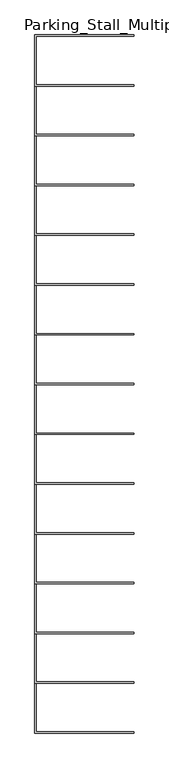
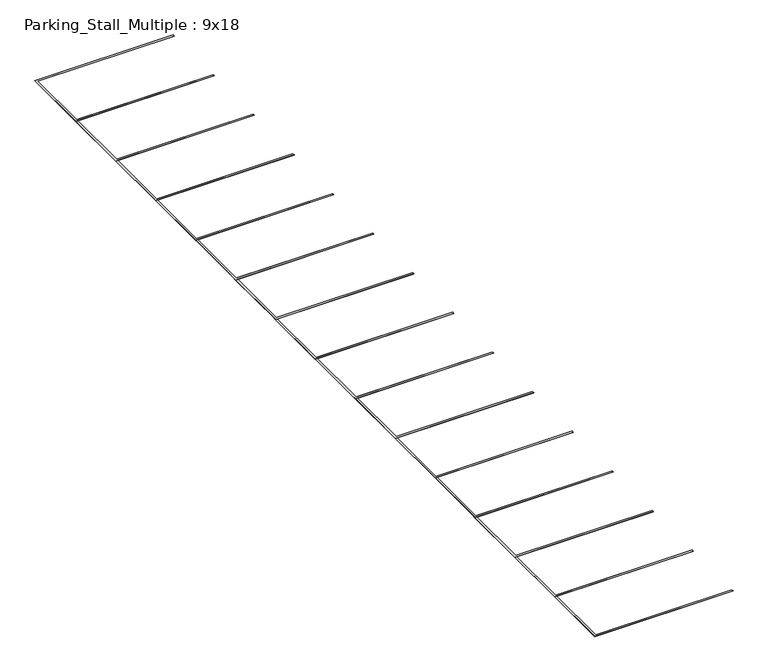
"""IFC4 building model written with IfcOpenShell, lengths in millimetres: proxy geometry, Parking_Stall_Multiple : 9x18."""

import ifcopenshell
import ifcopenshell.guid

model = None  # the IFC model being written
_history = None  # IfcOwnerHistory: only IFC2X3 demands one
_inside = {}  # id of a spatial element -> (the spatial element, [elements in it])
_under = {}  # id of a project, library or spatial element -> (it, [spatial elements below it])
_declared = {}  # id of a project -> (the project, [libraries it declares])
_typed = {}  # id of a type object -> (the type object, [elements of that type])
_made_of = {}  # id of a material, layer set ... -> (it, [elements and type objects made of it])


def new_model(schema):
    """Start an empty IFC model of exactly this schema.

    Asked for "IFC4X3", IfcOpenShell would pick the latest addendum, in which some entities
    have other attributes; the version numbers below select the first issue.
    IFC2X3 requires an IfcOwnerHistory on every rooted entity: one is made here for all.
    """
    global model, _history
    if schema == "IFC4X3":
        model = ifcopenshell.file(schema_version=(4, 3, 0, 0))
    else:
        model = ifcopenshell.file(schema=schema)
    _inside.clear()
    _under.clear()
    _declared.clear()
    _typed.clear()
    _made_of.clear()
    _history = None
    if model.schema == "IFC2X3":
        org = make("IfcOrganization", Name="unknown")
        user = make(
            "IfcPersonAndOrganization",
            ThePerson=make("IfcPerson", FamilyName="unknown"),
            TheOrganization=org,
        )
        app = make(
            "IfcApplication",
            ApplicationDeveloper=org,
            Version="unknown",
            ApplicationFullName="unknown",
            ApplicationIdentifier="unknown",
        )
        _history = make(
            "IfcOwnerHistory",
            OwningUser=user,
            OwningApplication=app,
            ChangeAction="ADDED",
            CreationDate=0,
        )
    return model


def make(cls, **values):
    """One entity of the class cls with the attributes given. An attribute that is None is left unset."""
    return model.create_entity(
        cls, **{name: value for name, value in values.items() if value is not None}
    )


def rooted(cls, **values):
    """An entity with a GlobalId (a new one), such as an element, a storey or a relation."""
    return make(cls, GlobalId=ifcopenshell.guid.new(), OwnerHistory=_history, **values)


def si_unit(unit_type, name, prefix=None):
    """IfcSIUnit, for example si_unit("LENGTHUNIT", "METRE", prefix="MILLI")."""
    return make("IfcSIUnit", UnitType=unit_type, Prefix=prefix, Name=name)


def assignment(units):
    """IfcUnitAssignment: the units of a project."""
    return None if units is None else make("IfcUnitAssignment", Units=units)


def point(xyz):
    """IfcCartesianPoint."""
    return None if xyz is None else make("IfcCartesianPoint", Coordinates=xyz)


def direction(xyz):
    """IfcDirection."""
    return None if xyz is None else make("IfcDirection", DirectionRatios=xyz)


def frame(location, z_axis=None, x_axis=None):
    """IfcAxis2Placement3D, a coordinate frame: its origin and axes. An axis left out is left unset."""
    return make(
        "IfcAxis2Placement3D",
        Location=point(location),
        Axis=direction(z_axis),
        RefDirection=direction(x_axis),
    )


def origin():
    """The frame at (0, 0, 0) with its axes left unset."""
    return frame((0.0, 0.0, 0.0))


def origin_with_axes():
    """The frame at (0, 0, 0) with the z axis (0, 0, 1) and the x axis (1, 0, 0) written out."""
    return frame((0.0, 0.0, 0.0), z_axis=(0.0, 0.0, 1.0), x_axis=(1.0, 0.0, 0.0))


def place(relative_to, where):
    """IfcLocalPlacement: puts the frame where relative to a parent placement (None: the world)."""
    return make(
        "IfcLocalPlacement", PlacementRelTo=relative_to, RelativePlacement=where
    )


def context(
    kind, dimensions, precision=None, world=None, true_north=None, identifier=None
):
    """IfcGeometricRepresentationContext, for example the 3D "Model" context."""
    return make(
        "IfcGeometricRepresentationContext",
        ContextIdentifier=identifier,
        ContextType=kind,
        CoordinateSpaceDimension=dimensions,
        Precision=precision,
        WorldCoordinateSystem=world,
        TrueNorth=true_north,
    )


def project(units=None, contexts=None):
    """IfcProject with its units and contexts."""
    return rooted(
        "IfcProject",
        Name="project",
        RepresentationContexts=contexts,
        UnitsInContext=assignment(units),
    )


def spatial(cls, under=None, at=None, **own):
    """A site, building, storey or space (cls), placed at a placement, below another one or the project."""
    s = rooted(cls, ObjectPlacement=at, **own)
    if under is not None:
        _under.setdefault(under.id(), (under, []))[1].append(s)
    return s


def polyline(points):
    """IfcPolyline through the points."""
    return make("IfcPolyline", Points=[point(p) for p in points])


def outline(outer, holes=None, kind="AREA"):
    """IfcArbitraryClosedProfileDef: a profile drawn as a closed curve; with holes, ...WithVoids."""
    if holes is None:
        return make("IfcArbitraryClosedProfileDef", ProfileType=kind, OuterCurve=outer)
    return make(
        "IfcArbitraryProfileDefWithVoids",
        ProfileType=kind,
        OuterCurve=outer,
        InnerCurves=holes,
    )


def extrude(swept, where, along, depth):
    """IfcExtrudedAreaSolid: the profile swept, set in the frame where, extruded along a direction by depth."""
    return make(
        "IfcExtrudedAreaSolid",
        SweptArea=swept,
        Position=where,
        ExtrudedDirection=direction(along),
        Depth=depth,
    )


def shape(context_of_items, identifier, shape_type, items):
    """IfcShapeRepresentation: the items that make up one representation, for example the "Body"."""
    return make(
        "IfcShapeRepresentation",
        ContextOfItems=context_of_items,
        RepresentationIdentifier=identifier,
        RepresentationType=shape_type,
        Items=items,
    )


def source(mapping_origin, context_of_items, identifier, shape_type, items):
    """IfcRepresentationMap: a shape defined once, which mapped items show again and again."""
    return make(
        "IfcRepresentationMap",
        MappingOrigin=mapping_origin,
        MappedRepresentation=shape(context_of_items, identifier, shape_type, items),
    )


def transform(
    local_origin,
    x_axis=None,
    y_axis=None,
    z_axis=None,
    scale=None,
    scale2=None,
    scale3=None,
    uniform=True,
):
    """IfcCartesianTransformationOperator3D, or its non-uniform kind. x_axis, y_axis, z_axis: its Axis1, 2, 3."""
    if uniform:
        return make(
            "IfcCartesianTransformationOperator3D",
            Axis1=direction(x_axis),
            Axis2=direction(y_axis),
            LocalOrigin=point(local_origin),
            Scale=scale,
            Axis3=direction(z_axis),
        )
    return make(
        "IfcCartesianTransformationOperator3DnonUniform",
        Axis1=direction(x_axis),
        Axis2=direction(y_axis),
        LocalOrigin=point(local_origin),
        Scale=scale,
        Axis3=direction(z_axis),
        Scale2=scale2,
        Scale3=scale3,
    )


def mapped(mapping_source, mapping_target):
    """IfcMappedItem: shows the shape of a source again, moved by a transform."""
    return make(
        "IfcMappedItem", MappingSource=mapping_source, MappingTarget=mapping_target
    )


def made_of(thing, what):
    """Note that an element or type object is made of a material, layer set ...; save() writes the relation."""
    if what is not None:
        _made_of.setdefault(what.id(), (what, []))[1].append(thing)
    return thing


def element(
    cls,
    number,
    at=None,
    inside=None,
    cuts=None,
    type_object=None,
    material=None,
    context=None,
    identifier="Body",
    shape_type=None,
    held_by="IfcProductDefinitionShape",
    body=None,
    shapes=None,
    **own,
):
    """One element of the class cls, such as IfcWall. Its Tag is "e" and its number.

    at: its placement. inside: the storey or other place that contains it. cuts: it is an
    opening in that element (IfcRelVoidsElement). A single representation is given by context,
    identifier, shape_type and body (its items); several are given by shapes. held_by: the class
    of the entity that holds the representations. save() writes the other relations.
    """
    e = rooted(cls, Tag="e%d" % number, ObjectPlacement=at, **own)
    if body is not None:
        shapes = [shape(context, identifier, shape_type, body)]
    if shapes is not None:
        e.Representation = make(held_by, Representations=shapes)
    if inside is not None:
        _inside.setdefault(inside.id(), (inside, []))[1].append(e)
    if cuts is not None:
        rooted(
            "IfcRelVoidsElement", RelatingBuildingElement=cuts, RelatedOpeningElement=e
        )
    if type_object is not None:
        _typed.setdefault(type_object.id(), (type_object, []))[1].append(e)
    return made_of(e, material)


def aggregate(whole, parts):
    """IfcRelAggregates: a whole, such as a stair, and the parts it consists of."""
    return rooted("IfcRelAggregates", RelatingObject=whole, RelatedObjects=parts)


def save(model, path):
    """Write the relations noted so far, then the file.

    IfcRelAggregates (storeys below a building ...), IfcRelContainedInSpatialStructure (elements
    in a storey), IfcRelDefinesByType, IfcRelAssociatesMaterial and IfcRelDeclares: one each for
    every whole, place, type object, material and project.
    """
    for whole, parts in _under.values():
        aggregate(whole, parts)
    for where, things in _inside.values():
        rooted(
            "IfcRelContainedInSpatialStructure",
            RelatedElements=things,
            RelatingStructure=where,
        )
    for kind, things in _typed.values():
        rooted("IfcRelDefinesByType", RelatedObjects=things, RelatingType=kind)
    for what, things in _made_of.values():
        rooted("IfcRelAssociatesMaterial", RelatedObjects=things, RelatingMaterial=what)
    for by, libraries in _declared.values():
        rooted("IfcRelDeclares", RelatingContext=by, RelatedDefinitions=libraries)
    model.write(path)


def parking_stall_multiple_9x18_4ba3b90c(model_context):
    return source(origin(), model_context, "Body", "SweptSolid", [
        extrude(outline(polyline([(5486.4, 35661.6), (0.0, 35661.6), (0.0, 38481.0), (5486.4, 38481.0), (5486.4, 38404.8), (76.2, 38404.8), (76.2, 35737.8), (5486.4, 35737.8), (5486.4, 35661.6)])), origin_with_axes(), (0.0, 0.0, 1.0), 6.35),
        extrude(outline(polyline([(5486.4, 32918.4), (0.0, 32918.4), (0.0, 35737.8), (5486.4, 35737.8), (5486.4, 35661.6), (76.2, 35661.6), (76.2, 32994.6), (5486.4, 32994.6), (5486.4, 32918.4)])), origin_with_axes(), (0.0, 0.0, 1.0), 6.35),
        extrude(outline(polyline([(5486.4, 30175.2), (0.0, 30175.2), (0.0, 32994.6), (5486.4, 32994.6), (5486.4, 32918.4), (76.2, 32918.4), (76.2, 30251.4), (5486.4, 30251.4), (5486.4, 30175.2)])), origin_with_axes(), (0.0, 0.0, 1.0), 6.35),
        extrude(outline(polyline([(5486.4, 27432.0), (0.0, 27432.0), (0.0, 30251.4), (5486.4, 30251.4), (5486.4, 30175.2), (76.2, 30175.2), (76.2, 27508.2), (5486.4, 27508.2), (5486.4, 27432.0)])), origin_with_axes(), (0.0, 0.0, 1.0), 6.35),
        extrude(outline(polyline([(5486.4, 24688.8), (0.0, 24688.8), (0.0, 27508.2), (5486.4, 27508.2), (5486.4, 27432.0), (76.2, 27432.0), (76.2, 24765.0), (5486.4, 24765.0), (5486.4, 24688.8)])), origin_with_axes(), (0.0, 0.0, 1.0), 6.35),
        extrude(outline(polyline([(5486.4, 21945.6), (0.0, 21945.6), (0.0, 24765.0), (5486.4, 24765.0), (5486.4, 24688.8), (76.2, 24688.8), (76.2, 22021.8), (5486.4, 22021.8), (5486.4, 21945.6)])), origin_with_axes(), (0.0, 0.0, 1.0), 6.35),
        extrude(outline(polyline([(5486.4, 19202.4), (0.0, 19202.4), (0.0, 22021.8), (5486.4, 22021.8), (5486.4, 21945.6), (76.2, 21945.6), (76.2, 19278.6), (5486.4, 19278.6), (5486.4, 19202.4)])), origin_with_axes(), (0.0, 0.0, 1.0), 6.35),
        extrude(outline(polyline([(5486.4, 16459.2), (0.0, 16459.2), (0.0, 19278.6), (5486.4, 19278.6), (5486.4, 19202.4), (76.2, 19202.4), (76.2, 16535.4), (5486.4, 16535.4), (5486.4, 16459.2)])), origin_with_axes(), (0.0, 0.0, 1.0), 6.35),
        extrude(outline(polyline([(5486.4, 13716.0), (0.0, 13716.0), (0.0, 16535.4), (5486.4, 16535.4), (5486.4, 16459.2), (76.2, 16459.2), (76.2, 13792.2), (5486.4, 13792.2), (5486.4, 13716.0)])), origin_with_axes(), (0.0, 0.0, 1.0), 6.35),
        extrude(outline(polyline([(5486.4, 10972.8), (0.0, 10972.8), (0.0, 13792.2), (5486.4, 13792.2), (5486.4, 13716.0), (76.2, 13716.0), (76.2, 11049.0), (5486.4, 11049.0), (5486.4, 10972.8)])), origin_with_axes(), (0.0, 0.0, 1.0), 6.35),
        extrude(outline(polyline([(5486.4, 8229.6), (0.0, 8229.6), (0.0, 11049.0), (5486.4, 11049.0), (5486.4, 10972.8), (76.2, 10972.8), (76.2, 8305.8), (5486.4, 8305.8), (5486.4, 8229.6)])), origin_with_axes(), (0.0, 0.0, 1.0), 6.35),
        extrude(outline(polyline([(5486.4, 5486.4), (0.0, 5486.4), (0.0, 8305.8), (5486.4, 8305.8), (5486.4, 8229.6), (76.2, 8229.6), (76.2, 5562.6), (5486.4, 5562.6), (5486.4, 5486.4)])), origin_with_axes(), (0.0, 0.0, 1.0), 6.35),
        extrude(outline(polyline([(5486.4, 2743.2), (0.0, 2743.2), (0.0, 5562.6), (5486.4, 5562.6), (5486.4, 5486.4), (76.2, 5486.4), (76.2, 2819.4), (5486.4, 2819.4), (5486.4, 2743.2)])), origin_with_axes(), (0.0, 0.0, 1.0), 6.35),
        extrude(outline(polyline([(5486.4, 0.0), (0.0, 0.0), (0.0, 2819.4), (5486.4, 2819.4), (5486.4, 2743.2), (76.2, 2743.2), (76.2, 76.2), (5486.4, 76.2), (5486.4, 0.0)])), origin_with_axes(), (0.0, 0.0, 1.0), 6.35),
    ])


if __name__ == "__main__":
    model = new_model("IFC4")
    model_context = context("Model", 3, world=origin())
    ifc_project = project(units=[si_unit("LENGTHUNIT", "METRE", prefix="MILLI")], contexts=[model_context])
    site = spatial("IfcSite", under=ifc_project)
    building = spatial("IfcBuilding", under=site)
    placement = place(None, origin())
    parking_stall_multiple_9x18_shape = parking_stall_multiple_9x18_4ba3b90c(model_context)
    element("IfcBuildingElementProxy", 1, Name="Parking_Stall_Multiple : 9x18", ObjectType="Parking_Stall_Multiple : 9x18", at=placement, inside=building, context=model_context, shape_type="MappedRepresentation", body=[
        mapped(parking_stall_multiple_9x18_shape, transform((0.0, 0.0, 0.0), x_axis=(1.0, 0.0, 0.0), y_axis=(0.0, 1.0, 0.0), z_axis=(0.0, 0.0, 1.0))),
    ])
    save(model, "model.ifc")

# Revit data of these elements
# Type "Parking_Stall_Multiple : 9x18"
#   Type Mark = "PK-1"
#   Parking_Width_M = 9' - 0"
#   Parking_Run_Length [instance default] = 65' - 0"
#   Parking_Line_Width = 0' - 3"
#   Parking_Length_M = 18' - 0"
#   Single_Parking_Visibility [instance default] = no
#   Parking_ADA_Symbol = no
#   ParkingUnitsArray [instance default] = 7
#   ParkingUnits [instance default] = 7
#   Multiple_Parking_Visibility [instance default] = yes
#   Parking_Line_Material = none
# Element 1 (IfcBuildingElementProxy, "Parking_Stall_Multiple : 9x18")
#   Parking_Run_Length = 125' - 0.51124"
#   ParkingUnitsArray = 14
#   ParkingUnits = 14
